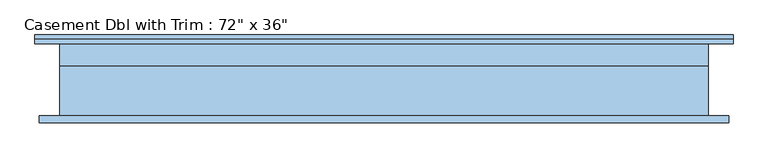
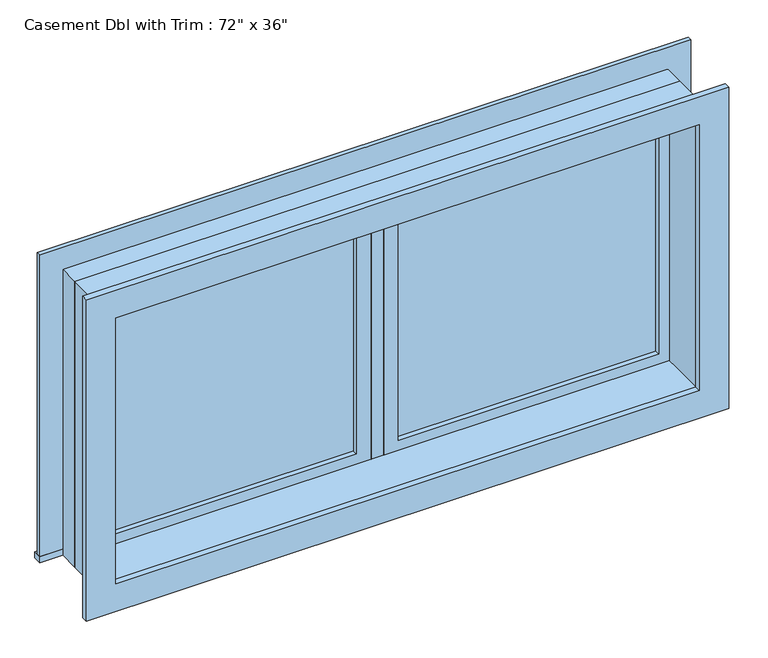
"""IFC4 building model written with IfcOpenShell, lengths in millimetres: window geometry."""

from ifc_helpers import new_model, si_unit, frame, origin, place, context, project, spatial, polyline, outline, extrude, source, transform, mapped, element, save


def window_193e8dfc(model_context):
    return source(origin(), model_context, "Body", "SweptSolid", [
        extrude(outline(polyline([(63.5, 85.725), (850.9, 85.725), (850.9, 73.025), (63.5, 73.025), (63.5, 85.725)])), frame((0.0, 0.0, 1282.7), z_axis=(0.0, 0.0, 1.0), x_axis=(1.0, 0.0, 0.0)), (0.0, 0.0, 1.0), 787.4),
        extrude(outline(polyline([(2114.55, 19.05), (1238.25, 19.05), (1238.25, 895.35), (2114.55, 895.35), (2114.55, 19.05)]), holes=[polyline([(2070.1, 63.5), (2070.1, 850.9), (1282.7, 850.9), (1282.7, 63.5), (2070.1, 63.5)])]), frame((0.0, 57.15, 0.0), z_axis=(0.0, 1.0, 0.0), x_axis=(0.0, 0.0, 1.0)), (0.0, 0.0, 1.0), 44.45),
        extrude(outline(polyline([(19.05, 57.15), (-19.05, 57.15), (-19.05, 120.65), (19.05, 120.65), (19.05, 57.15)])), frame((0.0, 0.0, 1238.25), z_axis=(0.0, 0.0, 1.0), x_axis=(1.0, 0.0, 0.0)), (0.0, 0.0, 1.0), 876.3),
        extrude(outline(polyline([(-984.25, 146.05), (984.25, 146.05), (984.25, 120.65), (-984.25, 120.65), (-984.25, 146.05)])), frame((0.0, 0.0, 1219.2), z_axis=(0.0, 0.0, 1.0), x_axis=(1.0, 0.0, 0.0)), (0.0, 0.0, 1.0), 19.05),
        extrude(outline(polyline([(2114.55, -895.35), (2114.55, 895.35), (1238.25, 895.35), (1238.25, 984.25), (2203.45, 984.25), (2203.45, -984.25), (1238.25, -984.25), (1238.25, -895.35), (2114.55, -895.35)])), frame((0.0, 120.65, 0.0), z_axis=(0.0, 1.0, 0.0), x_axis=(0.0, 0.0, 1.0)), (0.0, 0.0, 1.0), 12.7),
        extrude(outline(polyline([(2190.75, 971.55), (2190.75, -971.55), (1162.05, -971.55), (1162.05, 971.55), (2190.75, 971.55)]), holes=[polyline([(2101.85, 882.65), (1250.95, 882.65), (1250.95, -882.65), (2101.85, -882.65), (2101.85, 882.65)])]), frame((0.0, -101.6, 0.0), z_axis=(0.0, 1.0, 0.0), x_axis=(0.0, 0.0, 1.0)), (0.0, 0.0, 1.0), 19.05),
        extrude(outline(polyline([(-63.5, 73.025), (-850.9, 73.025), (-850.9, 85.725), (-63.5, 85.725), (-63.5, 73.025)])), frame((0.0, 0.0, 1282.7), z_axis=(0.0, 0.0, 1.0), x_axis=(1.0, 0.0, 0.0)), (0.0, 0.0, 1.0), 787.4),
        extrude(outline(polyline([(2114.55, -895.35), (1238.25, -895.35), (1238.25, -19.05), (2114.55, -19.05), (2114.55, -895.35)]), holes=[polyline([(2070.1, -850.9), (2070.1, -63.5), (1282.7, -63.5), (1282.7, -850.9), (2070.1, -850.9)])]), frame((0.0, 57.15, 0.0), z_axis=(0.0, 1.0, 0.0), x_axis=(0.0, 0.0, 1.0)), (0.0, 0.0, 1.0), 44.45),
        extrude(outline(polyline([(2133.6, -914.4), (1219.2, -914.4), (1219.2, 914.4), (2133.6, 914.4), (2133.6, -914.4)]), holes=[polyline([(2101.85, -882.65), (2101.85, 882.65), (1250.95, 882.65), (1250.95, -882.65), (2101.85, -882.65)])]), frame((0.0, -82.55, 0.0), z_axis=(0.0, 1.0, 0.0), x_axis=(0.0, 0.0, 1.0)), (0.0, 0.0, 1.0), 139.7),
        extrude(outline(polyline([(2133.6, 914.4), (2133.6, -914.4), (1219.2, -914.4), (1219.2, 914.4), (2133.6, 914.4)]), holes=[polyline([(2114.55, 895.35), (1238.25, 895.35), (1238.25, -895.35), (2114.55, -895.35), (2114.55, 895.35)])]), frame((0.0, 57.15, 0.0), z_axis=(0.0, 1.0, 0.0), x_axis=(0.0, 0.0, 1.0)), (0.0, 0.0, 1.0), 63.5),
    ])


if __name__ == "__main__":
    model = new_model("IFC4")
    model_context = context("Model", 3, world=origin())
    ifc_project = project(units=[si_unit("LENGTHUNIT", "METRE", prefix="MILLI")], contexts=[model_context])
    site = spatial("IfcSite", under=ifc_project)
    building = spatial("IfcBuilding", under=site)
    placement = place(None, origin())
    window_shape = window_193e8dfc(model_context)
    element("IfcWindow", 1, ObjectType="Casement Dbl with Trim : 72\" x 36\"", at=placement, inside=building, context=model_context, shape_type="MappedRepresentation", body=[
        mapped(window_shape, transform((0.0, 0.0, 0.0), x_axis=(1.0, 0.0, 0.0), y_axis=(0.0, 1.0, 0.0), z_axis=(0.0, 0.0, 1.0))),
    ])
    save(model, "model.ifc")

# Revit data of these elements
# Type "Casement Dbl with Trim : 72\" x 36\""
#   Type Mark = "11"
#   Construction Type Id = "GSP4R"
#   Assembly Code = "B2020100"
#   Analytic Construction = "1/8 in Pilkington single glazing"
#   Visual Light Transmittance = 0.9
#   Solar Heat Gain Coefficient = 0.78
#   Heat Transfer Coefficient (U) = 3.6886 W/(m²·K)
#   Height = 3' - 0"
#   Default Sill Height = 4' - 0"
#   Trim Projection - Ext. = 0' - 0 1/2"
#   Trim Projection - Int. = 0' - 0 3/4"
#   Trim Width - Exterior = 0' - 3 1/2"
#   Trim Width - Interior = 0' - 3 1/2"
#   Width = 6' - 0"
#   Window Inset = 0' - 0 3/4"
#   Glass Pane Material = Glass
#   Sash Material = Sash
#   Trim Exterior Material = Trim
#   Trim Interior Material = Trim
#   Wall Closure = (empty or 0)
# Element 1 (IfcWindow, "Casement Dbl with Trim : 72\" x 36\"")
#   Materials on its faces: "Sash", "Trim", "Glass"
# Materials
#   "Glass": class "Glass", colour RGB 0 128 192, transparency 0.75, Description = "Soda Lime Glass", Cost = 0
#   "Sash": class "Wood", colour RGB 224 178 126, transparency 0, Cost = 0
#   "Trim": class "Wood", colour RGB 224 178 126, transparency 0
